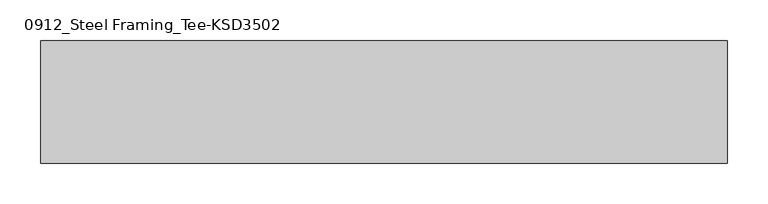
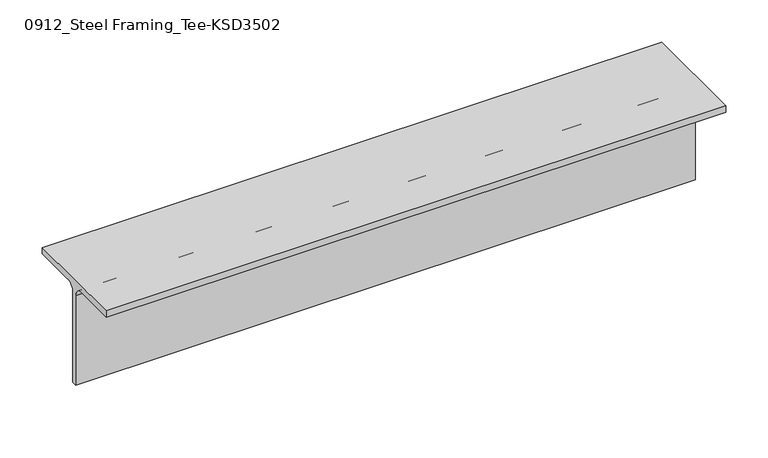
"""IFC4 building model written with IfcOpenShell, lengths in millimetres: member geometry, 0912_Steel Framing_Tee-KSD3502 : H_SB_ASB_CT-150x150x6.5x9."""

from ifc_helpers import new_model, si_unit, point, frame, frame_2d, origin, place, context, project, spatial, polyline, circle_curve, trimmed, segment, composite_curve, outline, extrude, source, transform, mapped, element, save


def member_0912_steel_framing_tee_ksd3502_e15e1797(model_context):
    return source(origin(), model_context, "Body", "SweptSolid", [
        extrude(outline(composite_curve([segment(polyline([(75.0, 75.0), (75.0, 66.0), (16.25, 66.0)]), True, "CONTINUOUS"), segment(trimmed(circle_curve(frame_2d((16.25, 53.0)), 13.0), [point((16.25, 66.0))], [point((3.25, 53.0))], True, "CARTESIAN"), True, "CONTINUOUS"), segment(polyline([(3.25, 53.0), (3.25, -75.0), (-3.25, -75.0), (-3.25, 53.0)]), True, "CONTINUOUS"), segment(trimmed(circle_curve(frame_2d((-16.25, 53.0)), 13.0), [point((-3.25, 53.0))], [point((-16.25, 66.0))], True, "CARTESIAN"), True, "CONTINUOUS"), segment(polyline([(-16.25, 66.0), (-75.0, 66.0), (-75.0, 75.0), (75.0, 75.0)]), True, "CONTINUOUS")], self_intersect=False)), frame((-500.0, 0.0, 0.0), z_axis=(1.0, 0.0, 0.0), x_axis=(0.0, 1.0, 0.0)), (0.0, 0.0, 1.0), 841.5),
    ])


if __name__ == "__main__":
    model = new_model("IFC4")
    model_context = context("Model", 3, world=origin())
    ifc_project = project(units=[si_unit("LENGTHUNIT", "METRE", prefix="MILLI")], contexts=[model_context])
    site = spatial("IfcSite", under=ifc_project)
    building = spatial("IfcBuilding", under=site)
    placement = place(None, origin())
    member_0912_steel_framing_tee_ksd3502_shape = member_0912_steel_framing_tee_ksd3502_e15e1797(model_context)
    element("IfcMember", 1, ObjectType="0912_Steel Framing_Tee-KSD3502 : H_SB_ASB_CT-150x150x6.5x9", at=placement, inside=building, context=model_context, shape_type="MappedRepresentation", body=[
        mapped(member_0912_steel_framing_tee_ksd3502_shape, transform((0.0, 0.0, 0.0), x_axis=(1.0, 0.0, 0.0), y_axis=(0.0, 1.0, 0.0), z_axis=(0.0, 0.0, 1.0))),
    ])
    save(model, "model.ifc")

# Revit data of these elements
# Type "0912_Steel Framing_Tee-KSD3502 : H_SB_ASB_CT-150x150x6.5x9"
#   H_WM Code_1 = "S01AA003-00001 | Main Steel Structure Fabrication Work | Shelter/Building | Light Steel - Standard (30KG/M>Weight) | Material: (   )"
#   H_WM Code_2 = "S03AA029-00001 | Main Steel Structure Erection Work | Shelter/Building | Light Steel (30KG/M>Weight) | Material: (   )"
#   H_WM Code_3 = "S01AA010-00001 | Main Steel Structure Fabrication Work | Shelter/Building | Steel Painting/Coating | for Non-Fireproofed Steel Surface, Surface Preparation, Primer, Second & Final Coat | Material: (   )"
#   H_Q'ty Cal Type Tag = "SB-Q2"
#   Width = 15.0 cm
#   Web Thickness = 0.65 cm
#   Web Fillet = 1.3 cm
#   Section Area = 23.39 cm²
#   Perimeter = 0.60 m²/m
#   Nominal Weight = 18.40 kgf/m
#   Height = 15.0 cm
#   Flange Thickness = 0.9 cm
#   Centroid Vertical = 7.5 cm
#   Centroid Horizontal = 7.5 cm
#   Length [instance default] = 1.5000 m
#   Structural Material [instance default] = Steel, 45-345
#   Warping Constant = (empty or 0)
#   Torsional Moment of Inertia = 0
#   Section Name Key = ""
#   Plastic Modulus weak axis = 0
#   Plastic Modulus strong axis = 0
#   Moment of Inertia weak axis = 0
#   Moment of Inertia strong axis = 0
#   Elastic Modulus weak axis = 0
#   Elastic Modulus strong axis = 0
#   Bolt Spacing = 0
#   Assembly Code = ""
# Element 1 (IfcMember, "0912_Steel Framing_Tee-KSD3502 : H_SB_ASB_CT-150x150x6.5x9")
#   Structural Material = none
# Materials
#   "Steel, 45-345": class "Metal", colour RGB 189 187 185, transparency 0, Description = "Steel 345 MPa", Cost = 0
